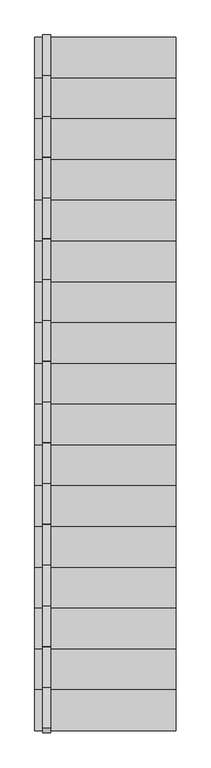
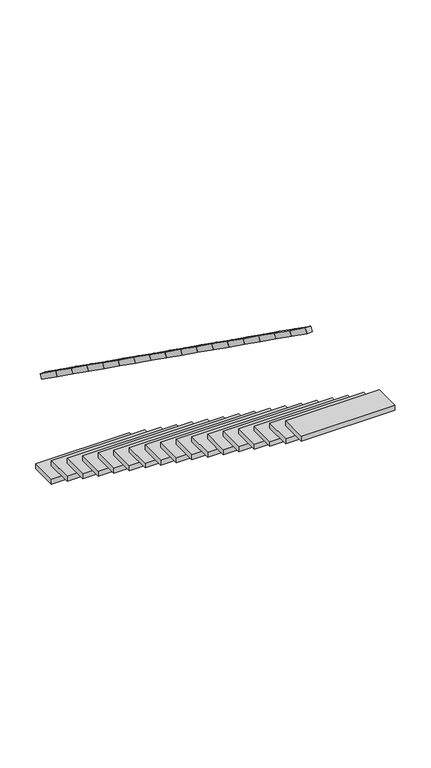
"""IFC4 building model written with IfcOpenShell, lengths in millimetres: stair geometry,   :  ."""

import ifcopenshell
import ifcopenshell.guid

model = None  # the IFC model being written
_history = None  # IfcOwnerHistory: only IFC2X3 demands one
_inside = {}  # id of a spatial element -> (the spatial element, [elements in it])
_under = {}  # id of a project, library or spatial element -> (it, [spatial elements below it])
_declared = {}  # id of a project -> (the project, [libraries it declares])
_typed = {}  # id of a type object -> (the type object, [elements of that type])
_made_of = {}  # id of a material, layer set ... -> (it, [elements and type objects made of it])


def new_model(schema):
    """Start an empty IFC model of exactly this schema.

    Asked for "IFC4X3", IfcOpenShell would pick the latest addendum, in which some entities
    have other attributes; the version numbers below select the first issue.
    IFC2X3 requires an IfcOwnerHistory on every rooted entity: one is made here for all.
    """
    global model, _history
    if schema == "IFC4X3":
        model = ifcopenshell.file(schema_version=(4, 3, 0, 0))
    else:
        model = ifcopenshell.file(schema=schema)
    _inside.clear()
    _under.clear()
    _declared.clear()
    _typed.clear()
    _made_of.clear()
    _history = None
    if model.schema == "IFC2X3":
        org = make("IfcOrganization", Name="unknown")
        user = make(
            "IfcPersonAndOrganization",
            ThePerson=make("IfcPerson", FamilyName="unknown"),
            TheOrganization=org,
        )
        app = make(
            "IfcApplication",
            ApplicationDeveloper=org,
            Version="unknown",
            ApplicationFullName="unknown",
            ApplicationIdentifier="unknown",
        )
        _history = make(
            "IfcOwnerHistory",
            OwningUser=user,
            OwningApplication=app,
            ChangeAction="ADDED",
            CreationDate=0,
        )
    return model


def make(cls, **values):
    """One entity of the class cls with the attributes given. An attribute that is None is left unset."""
    return model.create_entity(
        cls, **{name: value for name, value in values.items() if value is not None}
    )


def rooted(cls, **values):
    """An entity with a GlobalId (a new one), such as an element, a storey or a relation."""
    return make(cls, GlobalId=ifcopenshell.guid.new(), OwnerHistory=_history, **values)


def si_unit(unit_type, name, prefix=None):
    """IfcSIUnit, for example si_unit("LENGTHUNIT", "METRE", prefix="MILLI")."""
    return make("IfcSIUnit", UnitType=unit_type, Prefix=prefix, Name=name)


def assignment(units):
    """IfcUnitAssignment: the units of a project."""
    return None if units is None else make("IfcUnitAssignment", Units=units)


def point(xyz):
    """IfcCartesianPoint."""
    return None if xyz is None else make("IfcCartesianPoint", Coordinates=xyz)


def direction(xyz):
    """IfcDirection."""
    return None if xyz is None else make("IfcDirection", DirectionRatios=xyz)


def frame(location, z_axis=None, x_axis=None):
    """IfcAxis2Placement3D, a coordinate frame: its origin and axes. An axis left out is left unset."""
    return make(
        "IfcAxis2Placement3D",
        Location=point(location),
        Axis=direction(z_axis),
        RefDirection=direction(x_axis),
    )


def origin():
    """The frame at (0, 0, 0) with its axes left unset."""
    return frame((0.0, 0.0, 0.0))


def place(relative_to, where):
    """IfcLocalPlacement: puts the frame where relative to a parent placement (None: the world)."""
    return make(
        "IfcLocalPlacement", PlacementRelTo=relative_to, RelativePlacement=where
    )


def context(
    kind, dimensions, precision=None, world=None, true_north=None, identifier=None
):
    """IfcGeometricRepresentationContext, for example the 3D "Model" context."""
    return make(
        "IfcGeometricRepresentationContext",
        ContextIdentifier=identifier,
        ContextType=kind,
        CoordinateSpaceDimension=dimensions,
        Precision=precision,
        WorldCoordinateSystem=world,
        TrueNorth=true_north,
    )


def project(units=None, contexts=None):
    """IfcProject with its units and contexts."""
    return rooted(
        "IfcProject",
        Name="project",
        RepresentationContexts=contexts,
        UnitsInContext=assignment(units),
    )


def spatial(cls, under=None, at=None, **own):
    """A site, building, storey or space (cls), placed at a placement, below another one or the project."""
    s = rooted(cls, ObjectPlacement=at, **own)
    if under is not None:
        _under.setdefault(under.id(), (under, []))[1].append(s)
    return s


def polyline(points):
    """IfcPolyline through the points."""
    return make("IfcPolyline", Points=[point(p) for p in points])


def outline(outer, holes=None, kind="AREA"):
    """IfcArbitraryClosedProfileDef: a profile drawn as a closed curve; with holes, ...WithVoids."""
    if holes is None:
        return make("IfcArbitraryClosedProfileDef", ProfileType=kind, OuterCurve=outer)
    return make(
        "IfcArbitraryProfileDefWithVoids",
        ProfileType=kind,
        OuterCurve=outer,
        InnerCurves=holes,
    )


def extrude(swept, where, along, depth):
    """IfcExtrudedAreaSolid: the profile swept, set in the frame where, extruded along a direction by depth."""
    return make(
        "IfcExtrudedAreaSolid",
        SweptArea=swept,
        Position=where,
        ExtrudedDirection=direction(along),
        Depth=depth,
    )


def shape(context_of_items, identifier, shape_type, items):
    """IfcShapeRepresentation: the items that make up one representation, for example the "Body"."""
    return make(
        "IfcShapeRepresentation",
        ContextOfItems=context_of_items,
        RepresentationIdentifier=identifier,
        RepresentationType=shape_type,
        Items=items,
    )


def source(mapping_origin, context_of_items, identifier, shape_type, items):
    """IfcRepresentationMap: a shape defined once, which mapped items show again and again."""
    return make(
        "IfcRepresentationMap",
        MappingOrigin=mapping_origin,
        MappedRepresentation=shape(context_of_items, identifier, shape_type, items),
    )


def transform(
    local_origin,
    x_axis=None,
    y_axis=None,
    z_axis=None,
    scale=None,
    scale2=None,
    scale3=None,
    uniform=True,
):
    """IfcCartesianTransformationOperator3D, or its non-uniform kind. x_axis, y_axis, z_axis: its Axis1, 2, 3."""
    if uniform:
        return make(
            "IfcCartesianTransformationOperator3D",
            Axis1=direction(x_axis),
            Axis2=direction(y_axis),
            LocalOrigin=point(local_origin),
            Scale=scale,
            Axis3=direction(z_axis),
        )
    return make(
        "IfcCartesianTransformationOperator3DnonUniform",
        Axis1=direction(x_axis),
        Axis2=direction(y_axis),
        LocalOrigin=point(local_origin),
        Scale=scale,
        Axis3=direction(z_axis),
        Scale2=scale2,
        Scale3=scale3,
    )


def mapped(mapping_source, mapping_target):
    """IfcMappedItem: shows the shape of a source again, moved by a transform."""
    return make(
        "IfcMappedItem", MappingSource=mapping_source, MappingTarget=mapping_target
    )


def made_of(thing, what):
    """Note that an element or type object is made of a material, layer set ...; save() writes the relation."""
    if what is not None:
        _made_of.setdefault(what.id(), (what, []))[1].append(thing)
    return thing


def element(
    cls,
    number,
    at=None,
    inside=None,
    cuts=None,
    type_object=None,
    material=None,
    context=None,
    identifier="Body",
    shape_type=None,
    held_by="IfcProductDefinitionShape",
    body=None,
    shapes=None,
    **own,
):
    """One element of the class cls, such as IfcWall. Its Tag is "e" and its number.

    at: its placement. inside: the storey or other place that contains it. cuts: it is an
    opening in that element (IfcRelVoidsElement). A single representation is given by context,
    identifier, shape_type and body (its items); several are given by shapes. held_by: the class
    of the entity that holds the representations. save() writes the other relations.
    """
    e = rooted(cls, Tag="e%d" % number, ObjectPlacement=at, **own)
    if body is not None:
        shapes = [shape(context, identifier, shape_type, body)]
    if shapes is not None:
        e.Representation = make(held_by, Representations=shapes)
    if inside is not None:
        _inside.setdefault(inside.id(), (inside, []))[1].append(e)
    if cuts is not None:
        rooted(
            "IfcRelVoidsElement", RelatingBuildingElement=cuts, RelatedOpeningElement=e
        )
    if type_object is not None:
        _typed.setdefault(type_object.id(), (type_object, []))[1].append(e)
    return made_of(e, material)


def aggregate(whole, parts):
    """IfcRelAggregates: a whole, such as a stair, and the parts it consists of."""
    return rooted("IfcRelAggregates", RelatingObject=whole, RelatedObjects=parts)


def save(model, path):
    """Write the relations noted so far, then the file.

    IfcRelAggregates (storeys below a building ...), IfcRelContainedInSpatialStructure (elements
    in a storey), IfcRelDefinesByType, IfcRelAssociatesMaterial and IfcRelDeclares: one each for
    every whole, place, type object, material and project.
    """
    for whole, parts in _under.values():
        aggregate(whole, parts)
    for where, things in _inside.values():
        rooted(
            "IfcRelContainedInSpatialStructure",
            RelatedElements=things,
            RelatingStructure=where,
        )
    for kind, things in _typed.values():
        rooted("IfcRelDefinesByType", RelatedObjects=things, RelatingType=kind)
    for what, things in _made_of.values():
        rooted("IfcRelAssociatesMaterial", RelatedObjects=things, RelatingMaterial=what)
    for by, libraries in _declared.values():
        rooted("IfcRelDeclares", RelatingContext=by, RelatedDefinitions=libraries)
    model.write(path)


def stair_a78379cc(model_context):
    return source(origin(), model_context, "Body", "SweptSolid", [
        extrude(outline(polyline([(0.0, -319.1002977), (0.0, 0.0), (50.0, 0.0), (50.0, -319.1002977), (0.0, -319.1002977)])), frame((162072.7593015, 34520.3024209, 4178.947508), z_axis=(0.0, 0.5797550216229128, 0.8147908411997622), x_axis=(-1.0, 0.0, 0.0)), (0.0, 0.0, 1.0), 50.0),
        extrude(outline(polyline([(0.0, -319.1002977), (0.0, 0.0), (50.0, 0.0), (50.0, -319.1002977), (0.0, -319.1002977)])), frame((162072.7593015, 34780.3024209, 3993.947508), z_axis=(0.0, 0.5797550216228999, 0.8147908411997712), x_axis=(-1.0, 0.0, 0.0)), (0.0, 0.0, 1.0), 50.0),
        extrude(outline(polyline([(0.0, -319.1002977), (0.0, 0.0), (50.0, 0.0), (50.0, -319.1002977), (0.0, -319.1002977)])), frame((162072.7593015, 35040.3024209, 3808.947508), z_axis=(0.0, 0.5797550216229128, 0.8147908411997622), x_axis=(-1.0, 0.0, 0.0)), (0.0, 0.0, 1.0), 50.0),
        extrude(outline(polyline([(0.0, -319.1002977), (0.0, 0.0), (50.0, 0.0), (50.0, -319.1002977), (0.0, -319.1002977)])), frame((162072.7593015, 35300.3024209, 3623.947508), z_axis=(0.0, 0.5797550216229086, 0.8147908411997651), x_axis=(-1.0, 0.0, 0.0)), (0.0, 0.0, 1.0), 50.0),
        extrude(outline(polyline([(0.0, -319.1002977), (0.0, 0.0), (50.0, 0.0), (50.0, -319.1002977), (0.0, -319.1002977)])), frame((162072.7593015, 35560.3024209, 3438.947508), z_axis=(0.0, 0.5797550216229094, 0.8147908411997645), x_axis=(-1.0, 0.0, 0.0)), (0.0, 0.0, 1.0), 50.0),
        extrude(outline(polyline([(0.0, -319.1002977), (0.0, 0.0), (50.0, 0.0), (50.0, -319.1002977), (0.0, -319.1002977)])), frame((162072.7593015, 35820.3024209, 3253.947508), z_axis=(0.0, 0.5797550216229012, 0.8147908411997705), x_axis=(-1.0, 0.0, 0.0)), (0.0, 0.0, 1.0), 50.0),
        extrude(outline(polyline([(0.0, -319.1002977), (0.0, 0.0), (50.0, 0.0), (50.0, -319.1002977), (0.0, -319.1002977)])), frame((162072.7593015, 36080.3024209, 3068.947508), z_axis=(0.0, 0.5797550216229139, 0.8147908411997614), x_axis=(-1.0, 0.0, 0.0)), (0.0, 0.0, 1.0), 50.0),
        extrude(outline(polyline([(0.0, -319.1002977), (0.0, 0.0), (50.0, 0.0), (50.0, -319.1002977), (0.0, -319.1002977)])), frame((162072.7593015, 36340.3024209, 2883.947508), z_axis=(0.0, 0.579755021622915, 0.8147908411997605), x_axis=(-1.0, 0.0, 0.0)), (0.0, 0.0, 1.0), 50.0),
        extrude(outline(polyline([(0.0, -319.1002977), (0.0, 0.0), (50.0, 0.0), (50.0, -319.1002977), (0.0, -319.1002977)])), frame((162072.7593015, 36600.3024209, 2698.947508), z_axis=(0.0, 0.5797550216229116, 0.814790841199763), x_axis=(-1.0, 0.0, 0.0)), (0.0, 0.0, 1.0), 50.0),
        extrude(outline(polyline([(0.0, -319.1002977), (0.0, 0.0), (50.0, 0.0), (50.0, -319.1002977), (0.0, -319.1002977)])), frame((162072.7593015, 36860.3024209, 2513.947508), z_axis=(0.0, 0.5797550216228977, 0.8147908411997729), x_axis=(-1.0, 0.0, 0.0)), (0.0, 0.0, 1.0), 50.0),
        extrude(outline(polyline([(0.0, -319.1002977), (0.0, 0.0), (50.0, 0.0), (50.0, -319.1002977), (0.0, -319.1002977)])), frame((162072.7593015, 37120.3024209, 2328.947508), z_axis=(0.0, 0.5797550216229123, 0.8147908411997625), x_axis=(-1.0, 0.0, 0.0)), (0.0, 0.0, 1.0), 50.0),
        extrude(outline(polyline([(0.0, -319.1002977), (0.0, 0.0), (50.0, 0.0), (50.0, -319.1002977), (0.0, -319.1002977)])), frame((162072.7593015, 37380.3024209, 2143.947508), z_axis=(0.0, 0.5797550216229145, 0.814790841199761), x_axis=(-1.0, 0.0, 0.0)), (0.0, 0.0, 1.0), 50.0),
        extrude(outline(polyline([(0.0, -319.1002977), (0.0, 0.0), (50.0, 0.0), (50.0, -319.1002977), (0.0, -319.1002977)])), frame((162072.7593015, 37640.3024209, 1958.947508), z_axis=(0.0, 0.5797550216228994, 0.8147908411997717), x_axis=(-1.0, 0.0, 0.0)), (0.0, 0.0, 1.0), 50.0),
        extrude(outline(polyline([(0.0, -319.1002977), (0.0, 0.0), (50.0, 0.0), (50.0, -319.1002977), (0.0, -319.1002977)])), frame((162072.7593015, 37900.3024209, 1773.947508), z_axis=(0.0, 0.579755021622915, 0.8147908411997605), x_axis=(-1.0, 0.0, 0.0)), (0.0, 0.0, 1.0), 50.0),
        extrude(outline(polyline([(0.0, -319.1002977), (0.0, 0.0), (50.0, 0.0), (50.0, -319.1002977), (0.0, -319.1002977)])), frame((162072.7593015, 38160.3024209, 1588.947508), z_axis=(0.0, 0.5797550216229086, 0.8147908411997651), x_axis=(-1.0, 0.0, 0.0)), (0.0, 0.0, 1.0), 50.0),
        extrude(outline(polyline([(0.0, -319.1002977), (0.0, 0.0), (50.0, 0.0), (50.0, -319.1002977), (0.0, -319.1002977)])), frame((162072.7593015, 38420.3024209, 1403.947508), z_axis=(0.0, 0.5797550216229066, 0.8147908411997665), x_axis=(-1.0, 0.0, 0.0)), (0.0, 0.0, 1.0), 50.0),
        extrude(outline(polyline([(0.0, -319.1002977), (0.0, 0.0), (50.0, 0.0), (50.0, -319.1002977), (0.0, -319.1002977)])), frame((162072.7593015, 38680.3024209, 1218.947508), z_axis=(0.0, 0.5797550216228988, 0.8147908411997722), x_axis=(-1.0, 0.0, 0.0)), (0.0, 0.0, 1.0), 50.0),
        extrude(outline(polyline([(161972.7593015, 38694.7962965), (161972.7593015, 38954.7962965), (162872.7593015, 38954.7962965), (162872.7593015, 38694.7962965), (161972.7593015, 38694.7962965)])), frame((0.0, 0.0, 135.0), z_axis=(0.0, 0.0, 1.0), x_axis=(1.0, 0.0, 0.0)), (0.0, 0.0, 1.0), 50.0),
        extrude(outline(polyline([(161972.7593015, 38434.7962965), (161972.7593015, 38694.7962965), (162872.7593015, 38694.7962965), (162872.7593015, 38434.7962965), (161972.7593015, 38434.7962965)])), frame((0.0, 0.0, 320.0), z_axis=(0.0, 0.0, 1.0), x_axis=(1.0, 0.0, 0.0)), (0.0, 0.0, 1.0), 50.0),
        extrude(outline(polyline([(161972.7593015, 38174.7962965), (161972.7593015, 38434.7962965), (162872.7593015, 38434.7962965), (162872.7593015, 38174.7962965), (161972.7593015, 38174.7962965)])), frame((0.0, 0.0, 505.0), z_axis=(0.0, 0.0, 1.0), x_axis=(1.0, 0.0, 0.0)), (0.0, 0.0, 1.0), 50.0),
        extrude(outline(polyline([(161972.7593015, 37914.7962965), (161972.7593015, 38174.7962965), (162872.7593015, 38174.7962965), (162872.7593015, 37914.7962965), (161972.7593015, 37914.7962965)])), frame((0.0, 0.0, 690.0), z_axis=(0.0, 0.0, 1.0), x_axis=(1.0, 0.0, 0.0)), (0.0, 0.0, 1.0), 50.0),
        extrude(outline(polyline([(161972.7593015, 37654.7962965), (161972.7593015, 37914.7962965), (162872.7593015, 37914.7962965), (162872.7593015, 37654.7962965), (161972.7593015, 37654.7962965)])), frame((0.0, 0.0, 875.0), z_axis=(0.0, 0.0, 1.0), x_axis=(1.0, 0.0, 0.0)), (0.0, 0.0, 1.0), 50.0),
        extrude(outline(polyline([(161972.7593015, 37394.7962965), (161972.7593015, 37654.7962965), (162872.7593015, 37654.7962965), (162872.7593015, 37394.7962965), (161972.7593015, 37394.7962965)])), frame((0.0, 0.0, 1060.0), z_axis=(0.0, 0.0, 1.0), x_axis=(1.0, 0.0, 0.0)), (0.0, 0.0, 1.0), 50.0),
        extrude(outline(polyline([(161972.7593015, 37134.7962965), (161972.7593015, 37394.7962965), (162872.7593015, 37394.7962965), (162872.7593015, 37134.7962965), (161972.7593015, 37134.7962965)])), frame((0.0, 0.0, 1245.0), z_axis=(0.0, 0.0, 1.0), x_axis=(1.0, 0.0, 0.0)), (0.0, 0.0, 1.0), 50.0),
        extrude(outline(polyline([(161972.7593015, 36874.7962965), (161972.7593015, 37134.7962965), (162872.7593015, 37134.7962965), (162872.7593015, 36874.7962965), (161972.7593015, 36874.7962965)])), frame((0.0, 0.0, 1430.0), z_axis=(0.0, 0.0, 1.0), x_axis=(1.0, 0.0, 0.0)), (0.0, 0.0, 1.0), 50.0),
        extrude(outline(polyline([(161972.7593015, 36614.7962965), (161972.7593015, 36874.7962965), (162872.7593015, 36874.7962965), (162872.7593015, 36614.7962965), (161972.7593015, 36614.7962965)])), frame((0.0, 0.0, 1615.0), z_axis=(0.0, 0.0, 1.0), x_axis=(1.0, 0.0, 0.0)), (0.0, 0.0, 1.0), 50.0),
        extrude(outline(polyline([(161972.7593015, 36354.7962965), (161972.7593015, 36614.7962965), (162872.7593015, 36614.7962965), (162872.7593015, 36354.7962965), (161972.7593015, 36354.7962965)])), frame((0.0, 0.0, 1800.0), z_axis=(0.0, 0.0, 1.0), x_axis=(1.0, 0.0, 0.0)), (0.0, 0.0, 1.0), 50.0),
        extrude(outline(polyline([(161972.7593015, 36094.7962965), (161972.7593015, 36354.7962965), (162872.7593015, 36354.7962965), (162872.7593015, 36094.7962965), (161972.7593015, 36094.7962965)])), frame((0.0, 0.0, 1985.0), z_axis=(0.0, 0.0, 1.0), x_axis=(1.0, 0.0, 0.0)), (0.0, 0.0, 1.0), 50.0),
        extrude(outline(polyline([(161972.7593015, 35834.7962965), (161972.7593015, 36094.7962965), (162872.7593015, 36094.7962965), (162872.7593015, 35834.7962965), (161972.7593015, 35834.7962965)])), frame((0.0, 0.0, 2170.0), z_axis=(0.0, 0.0, 1.0), x_axis=(1.0, 0.0, 0.0)), (0.0, 0.0, 1.0), 50.0),
        extrude(outline(polyline([(161972.7593015, 35574.7962965), (161972.7593015, 35834.7962965), (162872.7593015, 35834.7962965), (162872.7593015, 35574.7962965), (161972.7593015, 35574.7962965)])), frame((0.0, 0.0, 2355.0), z_axis=(0.0, 0.0, 1.0), x_axis=(1.0, 0.0, 0.0)), (0.0, 0.0, 1.0), 50.0),
        extrude(outline(polyline([(161972.7593015, 35314.7962965), (161972.7593015, 35574.7962965), (162872.7593015, 35574.7962965), (162872.7593015, 35314.7962965), (161972.7593015, 35314.7962965)])), frame((0.0, 0.0, 2540.0), z_axis=(0.0, 0.0, 1.0), x_axis=(1.0, 0.0, 0.0)), (0.0, 0.0, 1.0), 50.0),
        extrude(outline(polyline([(161972.7593015, 35054.7962965), (161972.7593015, 35314.7962965), (162872.7593015, 35314.7962965), (162872.7593015, 35054.7962965), (161972.7593015, 35054.7962965)])), frame((0.0, 0.0, 2725.0), z_axis=(0.0, 0.0, 1.0), x_axis=(1.0, 0.0, 0.0)), (0.0, 0.0, 1.0), 50.0),
        extrude(outline(polyline([(161972.7593015, 34794.7962965), (161972.7593015, 35054.7962965), (162872.7593015, 35054.7962965), (162872.7593015, 34794.7962965), (161972.7593015, 34794.7962965)])), frame((0.0, 0.0, 2910.0), z_axis=(0.0, 0.0, 1.0), x_axis=(1.0, 0.0, 0.0)), (0.0, 0.0, 1.0), 50.0),
        extrude(outline(polyline([(161972.7593015, 34534.7962965), (161972.7593015, 34794.7962965), (162872.7593015, 34794.7962965), (162872.7593015, 34534.7962965), (161972.7593015, 34534.7962965)])), frame((0.0, 0.0, 3095.0), z_axis=(0.0, 0.0, 1.0), x_axis=(1.0, 0.0, 0.0)), (0.0, 0.0, 1.0), 50.0),
    ])


if __name__ == "__main__":
    model = new_model("IFC4")
    model_context = context("Model", 3, world=origin())
    ifc_project = project(units=[si_unit("LENGTHUNIT", "METRE", prefix="MILLI")], contexts=[model_context])
    site = spatial("IfcSite", under=ifc_project)
    building = spatial("IfcBuilding", under=site)
    placement = place(None, origin())
    stair_shape = stair_a78379cc(model_context)
    element("IfcStair", 1, ObjectType="  :  ", at=placement, inside=building, context=model_context, shape_type="MappedRepresentation", body=[
        mapped(stair_shape, transform((0.0, 0.0, 0.0), x_axis=(1.0, 0.0, 0.0), y_axis=(0.0, 1.0, 0.0), z_axis=(0.0, 0.0, 1.0))),
    ])
    save(model, "model.ifc")

# Revit data of these elements
# Type "  :  "
#   Abrechnungsart = "St"
#   Allright_Bauteil_ID = "0117Tre0000626342"
#   Material = "Stahlbeton"
#   Objektname = "Treppe"
#   NameOverride = " "
#   ThermalTransmittance = 0.0000 BTU/(h·ft²·°F)
#   NosingLength = 0.000 m
#   NumberOfRiser = 18
#   NumberOfTreads = 17
#   RiserHeight = 1.850 m
#   TreadLength = 2.600 m
#   IsExternal = no
#   FireExit = no
#   HandicapAccessible = no
#   HasNonSkidSurface = no
# Element 1 (IfcStair, "  :  ")
#   Materials on its faces: "*1", "weiss"
# Materials
#   "*1": class "Unassigned", colour RGB 175 175 175, transparency 0
#   "weiss": class "Unassigned", colour RGB 255 255 255, transparency 0
